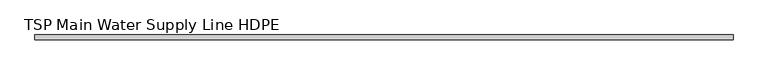
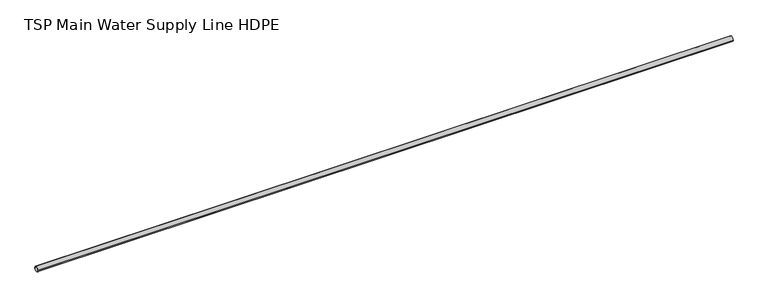
"""IFC4 building model written with IfcOpenShell, lengths in millimetres: flow terminal geometry, TSP Main Water Supply Line HDPE : HDPE Fresh Water Supply."""

from ifc_helpers import new_model, si_unit, point, frame, origin, origin_2d, place, context, project, spatial, circle_curve, trimmed, segment, composite_curve, outline, extrude, source, transform, mapped, element, save


def tsp_main_water_supply_line_hdpe_3eb8da9e(model_context):
    return source(origin(), model_context, "Body", "SweptSolid", [
        extrude(outline(composite_curve([segment(trimmed(circle_curve(origin_2d(), 16.0), [point((-16.0, 0.0))], [point((16.0, 0.0))], False, "CARTESIAN"), True, "CONTINUOUS"), segment(trimmed(circle_curve(origin_2d(), 16.0), [point((16.0, 0.0))], [point((-16.0, 0.0))], False, "CARTESIAN"), True, "CONTINUOUS")], self_intersect=False), holes=[composite_curve([segment(trimmed(circle_curve(origin_2d(), 15.0), [point((-15.0, 0.0))], [point((15.0, 0.0))], True, "CARTESIAN"), True, "CONTINUOUS"), segment(trimmed(circle_curve(origin_2d(), 15.0), [point((15.0, 0.0))], [point((-15.0, 0.0))], True, "CARTESIAN"), True, "CONTINUOUS")], self_intersect=False)]), frame((0.0, 0.0, 0.0), z_axis=(1.0, 0.0, 0.0), x_axis=(0.0, 1.0, 0.0)), (0.0, 0.0, 1.0), 4440.0),
    ])


if __name__ == "__main__":
    model = new_model("IFC4")
    model_context = context("Model", 3, world=origin())
    ifc_project = project(units=[si_unit("LENGTHUNIT", "METRE", prefix="MILLI")], contexts=[model_context])
    site = spatial("IfcSite", under=ifc_project)
    building = spatial("IfcBuilding", under=site)
    placement = place(None, origin())
    tsp_main_water_supply_line_hdpe_shape = tsp_main_water_supply_line_hdpe_3eb8da9e(model_context)
    element("IfcFlowTerminal", 1, ObjectType="TSP Main Water Supply Line HDPE : HDPE Fresh Water Supply", at=placement, inside=building, context=model_context, shape_type="MappedRepresentation", body=[
        mapped(tsp_main_water_supply_line_hdpe_shape, transform((0.0, 0.0, 0.0), x_axis=(1.0, 0.0, 0.0), y_axis=(0.0, 1.0, 0.0), z_axis=(0.0, 0.0, 1.0))),
    ])
    save(model, "model.ifc")

# Revit data of these elements
# Type "TSP Main Water Supply Line HDPE : HDPE Fresh Water Supply"
#   Model = "TSP_110SFWSP"
#   Pipe length [instance default] = 1200 mm
#   Pipe dia = 30 mm
#   built-in parameter 1001306 [instance default] = 3.93701 (stored number, unit not read)
#   Default Elevation = 0
# Element 1 (IfcFlowTerminal, "TSP Main Water Supply Line HDPE : HDPE Fresh Water Supply")
#   Pipe length = 4440 mm
#   built-in parameter 1001306 = 14.5669 (stored number, unit not read)
#   Materials on its faces: "Aluminum, Anodized Blue"
# Materials
#   "Aluminum, Anodized Blue": class "Metal", colour RGB 120 120 120, transparency 0, Description = "Anodized aluminum, blue", Cost = 0
